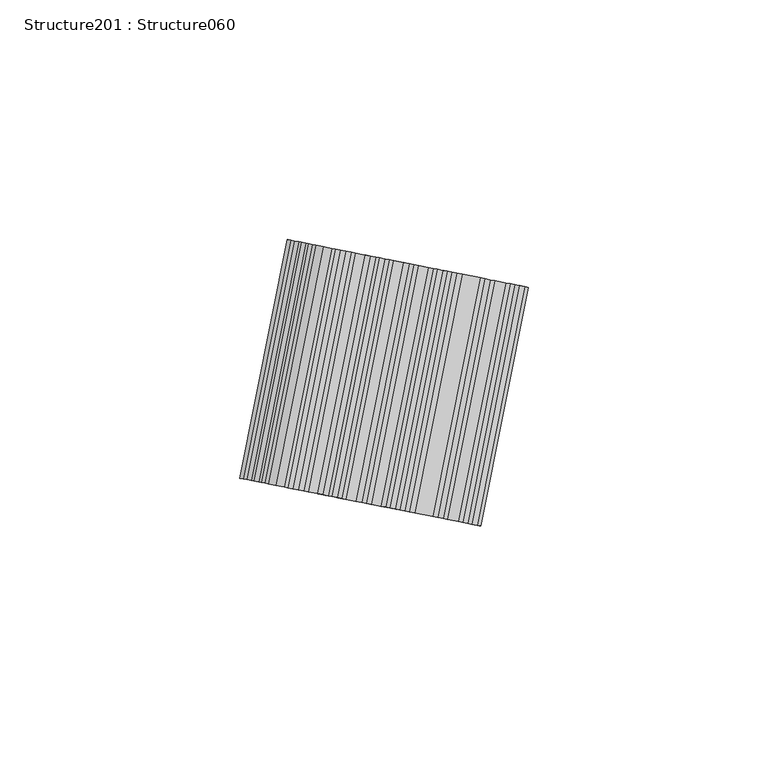
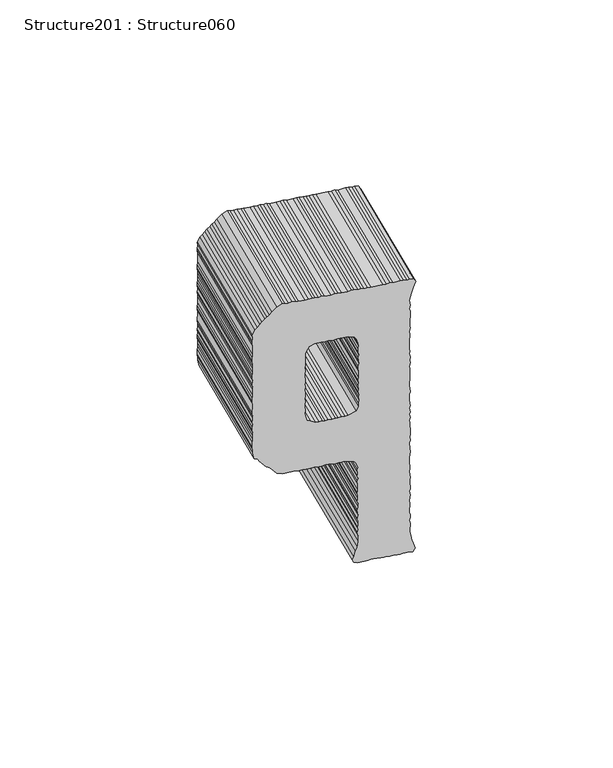
"""IFC4 building model written with IfcOpenShell, lengths in millimetres: proxy geometry, Structure201 : Structure060."""

from ifc_helpers import new_model, si_unit, frame, origin, place, context, project, spatial, polyline, outline, extrude, source, transform, mapped, element, save


def structure201_structure060_ac003c09(model_context):
    return source(origin(), model_context, "Body", "SweptSolid", [
        extrude(outline(polyline([(1.9520054, 0.0), (3.1183695, 0.256899), (4.0274788, 0.1273821), (5.3272739, 0.0), (7.4077287, 0.0), (8.3171938, 0.256899), (9.2263031, 0.0), (10.3976486, 0.256899), (11.1736828, 0.1273821), (12.3446725, 0.1273821), (13.5160181, 0.0), (15.463042, 0.1273821), (16.3725071, 0.1273821), (17.5434968, 0.256899), (18.7098609, 0.1273821), (19.7477756, 0.1273821), (20.5284353, 0.256899), (22.3470098, -0.5248282), (23.9086852, -1.9537844), (24.6847195, -2.8628937), (25.4703607, -3.5097668), (25.9894959, -4.1623329), (27.0270546, -4.9380113), (27.5461899, -5.7240084), (28.4552992, -6.6270688), (29.2363148, -7.2796349), (30.0119932, -8.9708273), (29.7550942, -10.1368356), (30.0119932, -11.3028439), (30.0119932, -12.0884851), (29.7550942, -13.2541376), (29.7550942, -16.2447692), (30.0119932, -17.2833954), (30.0119932, -18.5824788), (29.7550942, -19.4972812), (29.8835437, -20.4006974), (29.7550942, -21.4396795), (29.8835437, -22.7441001), (30.0119932, -23.6535653), (30.0119932, -24.6864985), (29.8835437, -25.7286829), (30.0119932, -27.0277663), (29.8835437, -28.0667483), (29.7550942, -28.9797716), (29.7550942, -31.0609381), (30.0119932, -32.0931596), (30.0119932, -33.264861), (29.7550942, -34.307757), (30.0119932, -37.425059), (29.8835437, -38.5932022), (29.7550942, -39.3731504), (30.0119932, -40.6722338), (29.8835437, -41.5777849), (30.0119932, -42.6199693), (30.0119932, -43.6585956), (29.8835437, -44.5680607), (29.7550942, -45.7376272), (29.8835437, -46.9096843), (30.0119932, -47.9479548), (30.0119932, -49.7665292), (29.7550942, -50.8090694), (29.7550942, -51.8455608), (29.3647643, -53.9228132), (28.3268497, -54.4458624), (27.8080703, -55.2218966), (26.2463949, -57.0401153), (25.5938287, -57.6926814), (24.55627, -58.2121724), (23.2564749, -59.7681548), (22.3470098, -60.8103392), (20.5284353, -61.4589914), (19.7477756, -61.3298302), (18.5814114, -61.1963993), (16.3725071, -61.1963993), (15.3345925, -61.4589914), (14.2920522, -61.3298302), (13.2541377, -61.4589914), (12.473122, -61.3298302), (11.1736828, -61.3298302), (10.2642177, -61.1963993), (9.0978536, -61.4589914), (8.3171938, -61.3298302), (7.0173988, -61.1963993), (5.0703749, -61.1963993), (3.8990293, -61.4589914), (2.98992, -61.3298302), (2.0804549, -61.3298302), (1.0425402, -61.1963993), (-0.2618804, -61.4589914), (-1.9470239, -61.9763475), (-2.4661591, -62.6289136), (-3.2468189, -64.320106), (-2.9849385, -65.2292153), (-3.1183694, -66.5243847), (-2.9849385, -67.566925), (-3.2468189, -68.4760343), (-2.9849385, -69.3854994), (-3.1183694, -70.6845828), (-3.1183694, -72.6362323), (-2.9849385, -73.6748586), (-3.1183694, -74.7134848), (-3.1183694, -75.7499762), (-2.9849385, -76.9216775), (-3.2468189, -77.7016257), (-3.2468189, -78.8694131), (-2.9849385, -79.9062602), (-3.1183694, -81.0818755), (-3.2468189, -81.9870709), (-2.9849385, -83.1587722), (-3.2468189, -83.9387204), (-3.2468189, -84.9773466), (-3.1183694, -86.270737), (-3.2468189, -87.0563782), (-2.9849385, -88.0950045), (-3.2468189, -89.3940879), (-3.2468189, -91.3421792), (-2.9849385, -93.4229899), (-2.3377096, -94.7163802), (-1.9470239, -96.7975467), (-1.4282445, -97.579274), (-1.9470239, -98.6157653), (-2.9849385, -98.8783574), (-5.1988242, -98.8783574), (-6.3651884, -98.7491962), (-7.2746535, -98.6157653), (-8.0553133, -98.6157653), (-10.3926671, -98.8783574), (-11.3021323, -98.8783574), (-12.3400468, -98.7491962), (-13.2491562, -98.8783574), (-14.2920522, -98.7491962), (-15.4584163, -98.8783574), (-16.5009565, -98.8783574), (-17.2769907, -98.7491962), (-19.4858951, -98.7491962), (-20.3953601, -98.8783574), (-21.17602, -97.579274), (-20.919121, -96.7975467), (-20.5287911, -95.7606995), (-20.0096559, -94.4594812), (-19.876225, -93.6798889), (-19.4858951, -91.3421792), (-19.4858951, -90.4327141), (-19.619326, -89.2667058), (-19.619326, -88.3519035), (-19.3574456, -87.3150563), (-19.619326, -86.1472689), (-19.619326, -85.2342456), (-19.3574456, -84.3286945), (-19.3574456, -83.2865101), (-19.4858951, -81.9870709), (-19.4858951, -81.0818755), (-19.3574456, -80.0393353), (-19.4858951, -79.130226), (-19.619326, -78.0876858), (-19.3574456, -76.7886024), (-19.619326, -75.8830513), (-19.619326, -74.970028), (-19.4858951, -73.9314017), (-19.4858951, -72.6362323), (-19.619326, -71.723209), (-19.4858951, -70.5572007), (-19.3574456, -69.5185745), (-19.4858951, -68.7386263), (-19.4858951, -67.7000001), (-19.3574456, -66.3952236), (-19.3574456, -64.4474881), (-19.4858951, -63.5380229), (-19.619326, -62.3684565), (-19.4858951, -61.1963993), (-19.3574456, -59.1212817), (-19.619326, -58.2121724), (-19.4858951, -57.0401153), (-19.619326, -56.136699), (-19.619326, -54.0558883), (-19.4858951, -53.1407302), (-19.4858951, -51.9747219), (-19.3574456, -50.9364514), (-19.619326, -49.8939112), (-19.3574456, -48.8570641), (-19.619326, -47.9479548), (-19.3574456, -46.6470923), (-19.619326, -45.6102451), (-19.4858951, -44.8285179), (-19.3574456, -43.5294345), (-19.3574456, -41.5777849), (-19.619326, -40.6722338), (-19.4858951, -39.3731504), (-19.3574456, -38.3302544), (-19.3574456, -37.2919839), (-19.4858951, -36.2551368), (-19.4858951, -32.2265905), (-19.3574456, -31.3135673), (-19.619326, -30.1457799), (-19.4858951, -29.2363148), (-19.619326, -27.9372314), (-19.3574456, -26.90074), (-19.4858951, -25.9916307), (-19.3574456, -25.0803865), (-19.3574456, -21.7001367), (-19.4858951, -20.6632895), (-19.4858951, -19.8812064), (-19.3574456, -18.71164), (-19.619326, -17.5438526), (-19.4858951, -16.6343875), (-19.4858951, -14.4258389), (-19.619326, -13.5170855), (-19.619326, -11.4362748), (-19.3574456, -10.5268097), (-19.619326, -9.2334193), (-19.3574456, -7.4091519), (-19.876225, -5.0714422), (-20.2665549, -4.032816), (-20.5287911, -2.9959688), (-20.919121, -2.2142415), (-21.3044695, -1.0443193), (-20.5287911, 0.1273821), (-19.3574456, 0.256899), (-18.4479804, 0.0), (-17.4104217, 0.256899), (-16.5009565, 0.256899), (-14.1636027, 0.0), (-13.2491562, 0.256899), (-12.082792, 0.0), (-11.0452333, 0.1273821), (-7.2746535, 0.0), (-6.1082894, 0.1273821), (-5.0653934, 0.0), (-4.0278345, 0.1273821), (-3.1183694, 0.0), (-1.9470239, 0.256899), (-1.0379145, 0.256899), (0.0, 0.0), (1.9520054, 0.0)]), holes=[polyline([(-2.59959, -43.6585956), (0.0, -44.8285179), (0.9091094, -44.9580348), (2.0804549, -44.8285179), (3.1183695, -44.9580348), (3.8990293, -44.9580348), (5.0703749, -45.085061), (6.2367389, -44.9580348), (7.2742978, -45.085061), (8.0553133, -44.9580348), (9.0978536, -45.085061), (10.2642177, -44.9580348), (11.8258932, -44.1816448), (12.7353582, -43.7916707), (13.1207067, -41.9734521), (13.3825872, -41.1917248), (13.1207067, -39.8926414), (13.3825872, -38.8536594), (13.3825872, -37.8168122), (13.2541377, -36.7728487), (13.3825872, -35.7360015), (13.2541377, -34.8211992), (13.1207067, -33.784352), (13.3825872, -32.7460816), (13.1207067, -31.5743802), (13.3825872, -30.7979902), (13.2541377, -29.7558058), (13.2541377, -28.8463407), (13.3825872, -27.8094935), (13.3825872, -26.6377922), (13.1207067, -25.5995217), (13.3825872, -24.4331576), (13.1207067, -23.6535653), (13.2541377, -22.4818639), (13.1207067, -21.3101626), (13.2541377, -20.4006974), (13.1207067, -19.3645619), (12.473122, -17.9356058), (12.0877735, -17.1538785), (10.3976486, -16.5016682), (8.3171938, -16.5016682), (7.0173988, -16.6343875), (6.1082894, -16.3739303), (4.9369439, -16.6343875), (4.1609097, -16.5016682), (3.1183695, -16.3739303), (-0.1284495, -16.3739303), (-2.0754734, -17.0264964), (-2.7280395, -17.8060888), (-3.1183694, -19.3645619), (-3.2468189, -20.4006974), (-3.1183694, -21.4396795), (-3.1183694, -22.6152948), (-3.3752684, -23.6535653), (-3.1183694, -24.4331576), (-3.2468189, -25.7286829), (-3.3752684, -26.6377922), (-3.1183694, -27.6806882), (-3.1183694, -28.5897975), (-3.2468189, -29.6223749), (-3.2468189, -31.7031855), (-3.1183694, -32.8791567), (-3.2468189, -33.6555467), (-3.1183694, -34.8211992), (-3.2468189, -35.9989494), (-3.1183694, -36.9023656), (-3.3752684, -38.0680181), (-3.2468189, -38.8536594), (-3.3752684, -39.8926414), (-3.2468189, -41.1917248), (-3.2468189, -42.2299952), (-2.59959, -43.6585956)])]), frame((-2299.8983794, 234924.9126584, 485.2778019), z_axis=(0.19466222296394123, 0.9808703374813293, 0.0), x_axis=(-0.9808703374813293, 0.19466222296394123, 0.0)), (0.0, 0.0, 1.0), 50.8),
    ])


if __name__ == "__main__":
    model = new_model("IFC4")
    model_context = context("Model", 3, world=origin())
    ifc_project = project(units=[si_unit("LENGTHUNIT", "METRE", prefix="MILLI")], contexts=[model_context])
    site = spatial("IfcSite", under=ifc_project)
    building = spatial("IfcBuilding", under=site)
    placement = place(None, origin())
    structure201_structure060_shape = structure201_structure060_ac003c09(model_context)
    element("IfcBuildingElementProxy", 1, Name="Structure201 : Structure060", ObjectType="Structure201 : Structure060", at=placement, inside=building, context=model_context, shape_type="MappedRepresentation", body=[
        mapped(structure201_structure060_shape, transform((0.0, 0.0, 0.0), x_axis=(1.0, 0.0, 0.0), y_axis=(0.0, 1.0, 0.0), z_axis=(0.0, 0.0, 1.0))),
    ])
    save(model, "model.ifc")

# Revit data of these elements
# Type "Structure201 : Structure060"
#   NameOverride = "Structure060"
# Element 1 (IfcBuildingElementProxy, "Structure201 : Structure060")
#   Materials on its faces: "BRUSHED ALUMINUM LETTERING"
# Materials
#   "BRUSHED ALUMINUM LETTERING": class "Unassigned", colour RGB 169 181 186, transparency 0, Cost = 0
